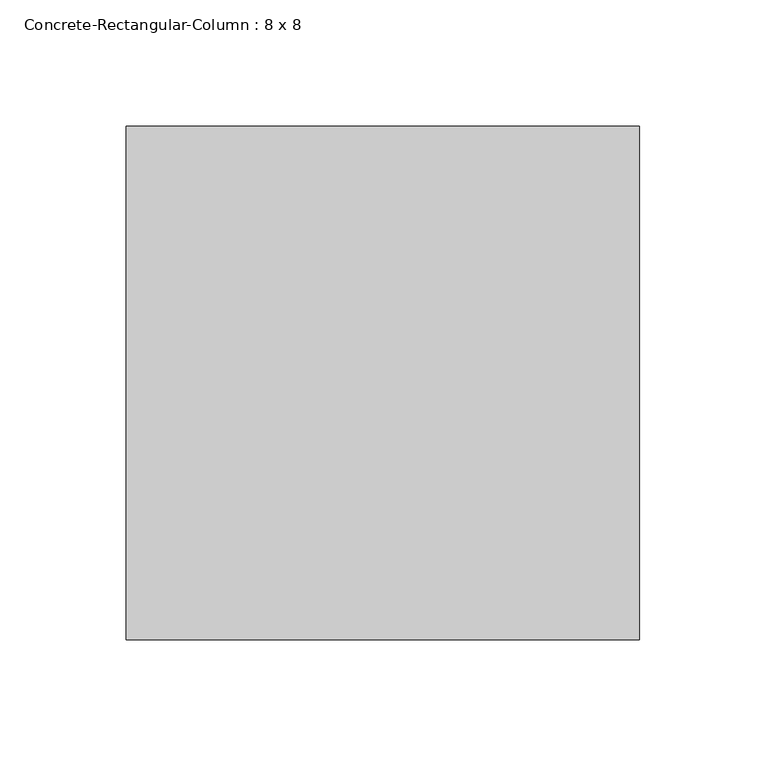
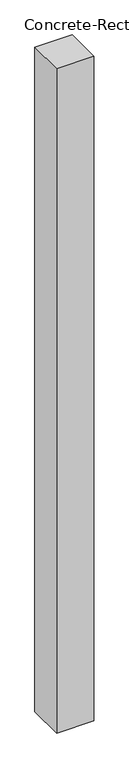
"""IFC4 building model written with IfcOpenShell, lengths in millimetres: column geometry, Concrete-Rectangular-Column : 8 x 8."""

import ifcopenshell
import ifcopenshell.guid

model = None  # the IFC model being written
_history = None  # IfcOwnerHistory: only IFC2X3 demands one
_inside = {}  # id of a spatial element -> (the spatial element, [elements in it])
_under = {}  # id of a project, library or spatial element -> (it, [spatial elements below it])
_declared = {}  # id of a project -> (the project, [libraries it declares])
_typed = {}  # id of a type object -> (the type object, [elements of that type])
_made_of = {}  # id of a material, layer set ... -> (it, [elements and type objects made of it])


def new_model(schema):
    """Start an empty IFC model of exactly this schema.

    Asked for "IFC4X3", IfcOpenShell would pick the latest addendum, in which some entities
    have other attributes; the version numbers below select the first issue.
    IFC2X3 requires an IfcOwnerHistory on every rooted entity: one is made here for all.
    """
    global model, _history
    if schema == "IFC4X3":
        model = ifcopenshell.file(schema_version=(4, 3, 0, 0))
    else:
        model = ifcopenshell.file(schema=schema)
    _inside.clear()
    _under.clear()
    _declared.clear()
    _typed.clear()
    _made_of.clear()
    _history = None
    if model.schema == "IFC2X3":
        org = make("IfcOrganization", Name="unknown")
        user = make(
            "IfcPersonAndOrganization",
            ThePerson=make("IfcPerson", FamilyName="unknown"),
            TheOrganization=org,
        )
        app = make(
            "IfcApplication",
            ApplicationDeveloper=org,
            Version="unknown",
            ApplicationFullName="unknown",
            ApplicationIdentifier="unknown",
        )
        _history = make(
            "IfcOwnerHistory",
            OwningUser=user,
            OwningApplication=app,
            ChangeAction="ADDED",
            CreationDate=0,
        )
    return model


def make(cls, **values):
    """One entity of the class cls with the attributes given. An attribute that is None is left unset."""
    return model.create_entity(
        cls, **{name: value for name, value in values.items() if value is not None}
    )


def rooted(cls, **values):
    """An entity with a GlobalId (a new one), such as an element, a storey or a relation."""
    return make(cls, GlobalId=ifcopenshell.guid.new(), OwnerHistory=_history, **values)


def si_unit(unit_type, name, prefix=None):
    """IfcSIUnit, for example si_unit("LENGTHUNIT", "METRE", prefix="MILLI")."""
    return make("IfcSIUnit", UnitType=unit_type, Prefix=prefix, Name=name)


def assignment(units):
    """IfcUnitAssignment: the units of a project."""
    return None if units is None else make("IfcUnitAssignment", Units=units)


def point(xyz):
    """IfcCartesianPoint."""
    return None if xyz is None else make("IfcCartesianPoint", Coordinates=xyz)


def direction(xyz):
    """IfcDirection."""
    return None if xyz is None else make("IfcDirection", DirectionRatios=xyz)


def frame(location, z_axis=None, x_axis=None):
    """IfcAxis2Placement3D, a coordinate frame: its origin and axes. An axis left out is left unset."""
    return make(
        "IfcAxis2Placement3D",
        Location=point(location),
        Axis=direction(z_axis),
        RefDirection=direction(x_axis),
    )


def origin():
    """The frame at (0, 0, 0) with its axes left unset."""
    return frame((0.0, 0.0, 0.0))


def origin_with_axes():
    """The frame at (0, 0, 0) with the z axis (0, 0, 1) and the x axis (1, 0, 0) written out."""
    return frame((0.0, 0.0, 0.0), z_axis=(0.0, 0.0, 1.0), x_axis=(1.0, 0.0, 0.0))


def place(relative_to, where):
    """IfcLocalPlacement: puts the frame where relative to a parent placement (None: the world)."""
    return make(
        "IfcLocalPlacement", PlacementRelTo=relative_to, RelativePlacement=where
    )


def context(
    kind, dimensions, precision=None, world=None, true_north=None, identifier=None
):
    """IfcGeometricRepresentationContext, for example the 3D "Model" context."""
    return make(
        "IfcGeometricRepresentationContext",
        ContextIdentifier=identifier,
        ContextType=kind,
        CoordinateSpaceDimension=dimensions,
        Precision=precision,
        WorldCoordinateSystem=world,
        TrueNorth=true_north,
    )


def project(units=None, contexts=None):
    """IfcProject with its units and contexts."""
    return rooted(
        "IfcProject",
        Name="project",
        RepresentationContexts=contexts,
        UnitsInContext=assignment(units),
    )


def spatial(cls, under=None, at=None, **own):
    """A site, building, storey or space (cls), placed at a placement, below another one or the project."""
    s = rooted(cls, ObjectPlacement=at, **own)
    if under is not None:
        _under.setdefault(under.id(), (under, []))[1].append(s)
    return s


def polyline(points):
    """IfcPolyline through the points."""
    return make("IfcPolyline", Points=[point(p) for p in points])


def outline(outer, holes=None, kind="AREA"):
    """IfcArbitraryClosedProfileDef: a profile drawn as a closed curve; with holes, ...WithVoids."""
    if holes is None:
        return make("IfcArbitraryClosedProfileDef", ProfileType=kind, OuterCurve=outer)
    return make(
        "IfcArbitraryProfileDefWithVoids",
        ProfileType=kind,
        OuterCurve=outer,
        InnerCurves=holes,
    )


def extrude(swept, where, along, depth):
    """IfcExtrudedAreaSolid: the profile swept, set in the frame where, extruded along a direction by depth."""
    return make(
        "IfcExtrudedAreaSolid",
        SweptArea=swept,
        Position=where,
        ExtrudedDirection=direction(along),
        Depth=depth,
    )


def shape(context_of_items, identifier, shape_type, items):
    """IfcShapeRepresentation: the items that make up one representation, for example the "Body"."""
    return make(
        "IfcShapeRepresentation",
        ContextOfItems=context_of_items,
        RepresentationIdentifier=identifier,
        RepresentationType=shape_type,
        Items=items,
    )


def source(mapping_origin, context_of_items, identifier, shape_type, items):
    """IfcRepresentationMap: a shape defined once, which mapped items show again and again."""
    return make(
        "IfcRepresentationMap",
        MappingOrigin=mapping_origin,
        MappedRepresentation=shape(context_of_items, identifier, shape_type, items),
    )


def transform(
    local_origin,
    x_axis=None,
    y_axis=None,
    z_axis=None,
    scale=None,
    scale2=None,
    scale3=None,
    uniform=True,
):
    """IfcCartesianTransformationOperator3D, or its non-uniform kind. x_axis, y_axis, z_axis: its Axis1, 2, 3."""
    if uniform:
        return make(
            "IfcCartesianTransformationOperator3D",
            Axis1=direction(x_axis),
            Axis2=direction(y_axis),
            LocalOrigin=point(local_origin),
            Scale=scale,
            Axis3=direction(z_axis),
        )
    return make(
        "IfcCartesianTransformationOperator3DnonUniform",
        Axis1=direction(x_axis),
        Axis2=direction(y_axis),
        LocalOrigin=point(local_origin),
        Scale=scale,
        Axis3=direction(z_axis),
        Scale2=scale2,
        Scale3=scale3,
    )


def mapped(mapping_source, mapping_target):
    """IfcMappedItem: shows the shape of a source again, moved by a transform."""
    return make(
        "IfcMappedItem", MappingSource=mapping_source, MappingTarget=mapping_target
    )


def made_of(thing, what):
    """Note that an element or type object is made of a material, layer set ...; save() writes the relation."""
    if what is not None:
        _made_of.setdefault(what.id(), (what, []))[1].append(thing)
    return thing


def element(
    cls,
    number,
    at=None,
    inside=None,
    cuts=None,
    type_object=None,
    material=None,
    context=None,
    identifier="Body",
    shape_type=None,
    held_by="IfcProductDefinitionShape",
    body=None,
    shapes=None,
    **own,
):
    """One element of the class cls, such as IfcWall. Its Tag is "e" and its number.

    at: its placement. inside: the storey or other place that contains it. cuts: it is an
    opening in that element (IfcRelVoidsElement). A single representation is given by context,
    identifier, shape_type and body (its items); several are given by shapes. held_by: the class
    of the entity that holds the representations. save() writes the other relations.
    """
    e = rooted(cls, Tag="e%d" % number, ObjectPlacement=at, **own)
    if body is not None:
        shapes = [shape(context, identifier, shape_type, body)]
    if shapes is not None:
        e.Representation = make(held_by, Representations=shapes)
    if inside is not None:
        _inside.setdefault(inside.id(), (inside, []))[1].append(e)
    if cuts is not None:
        rooted(
            "IfcRelVoidsElement", RelatingBuildingElement=cuts, RelatedOpeningElement=e
        )
    if type_object is not None:
        _typed.setdefault(type_object.id(), (type_object, []))[1].append(e)
    return made_of(e, material)


def aggregate(whole, parts):
    """IfcRelAggregates: a whole, such as a stair, and the parts it consists of."""
    return rooted("IfcRelAggregates", RelatingObject=whole, RelatedObjects=parts)


def save(model, path):
    """Write the relations noted so far, then the file.

    IfcRelAggregates (storeys below a building ...), IfcRelContainedInSpatialStructure (elements
    in a storey), IfcRelDefinesByType, IfcRelAssociatesMaterial and IfcRelDeclares: one each for
    every whole, place, type object, material and project.
    """
    for whole, parts in _under.values():
        aggregate(whole, parts)
    for where, things in _inside.values():
        rooted(
            "IfcRelContainedInSpatialStructure",
            RelatedElements=things,
            RelatingStructure=where,
        )
    for kind, things in _typed.values():
        rooted("IfcRelDefinesByType", RelatedObjects=things, RelatingType=kind)
    for what, things in _made_of.values():
        rooted("IfcRelAssociatesMaterial", RelatedObjects=things, RelatingMaterial=what)
    for by, libraries in _declared.values():
        rooted("IfcRelDeclares", RelatingContext=by, RelatedDefinitions=libraries)
    model.write(path)


def concrete_rectangular_column_8_x_8_f215429a(model_context):
    return source(origin(), model_context, "Body", "SweptSolid", [
        extrude(outline(polyline([(101.6, 101.6), (101.6, -101.6), (-101.6, -101.6), (-101.6, 101.6), (101.6, 101.6)])), origin_with_axes(), (0.0, 0.0, 1.0), 3810.0),
    ])


if __name__ == "__main__":
    model = new_model("IFC4")
    model_context = context("Model", 3, world=origin())
    ifc_project = project(units=[si_unit("LENGTHUNIT", "METRE", prefix="MILLI")], contexts=[model_context])
    site = spatial("IfcSite", under=ifc_project)
    building = spatial("IfcBuilding", under=site)
    placement = place(None, origin())
    concrete_rectangular_column_8_x_8_shape = concrete_rectangular_column_8_x_8_f215429a(model_context)
    element("IfcColumn", 1, ObjectType="Concrete-Rectangular-Column : 8 x 8", at=placement, inside=building, context=model_context, shape_type="MappedRepresentation", body=[
        mapped(concrete_rectangular_column_8_x_8_shape, transform((0.0, 0.0, 0.0), x_axis=(1.0, 0.0, 0.0), y_axis=(0.0, 1.0, 0.0), z_axis=(0.0, 0.0, 1.0))),
    ])
    save(model, "model.ifc")

# Revit data of these elements
# Type "Concrete-Rectangular-Column : 8 x 8"
#   Assembly Code = "B10"
#   b = 203.2 mm
#   h = 203.2 mm
#   Structural Material [instance default] = Concrete - Cast-in-Place Concrete
# Element 1 (IfcColumn, "Concrete-Rectangular-Column : 8 x 8")
#   Materials on its faces: "Concrete - Cast-in-Place Concrete"
# Materials
#   "Concrete - Cast-in-Place Concrete": class "Concrete", colour RGB 192 192 192, transparency 0
